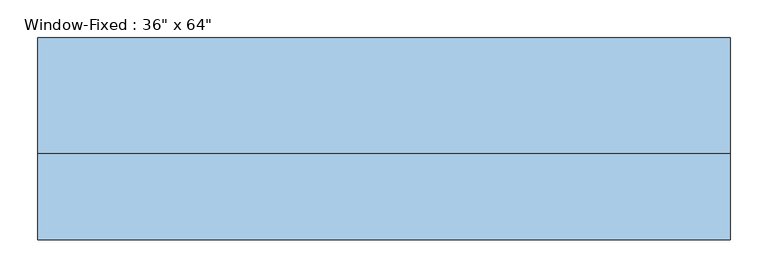
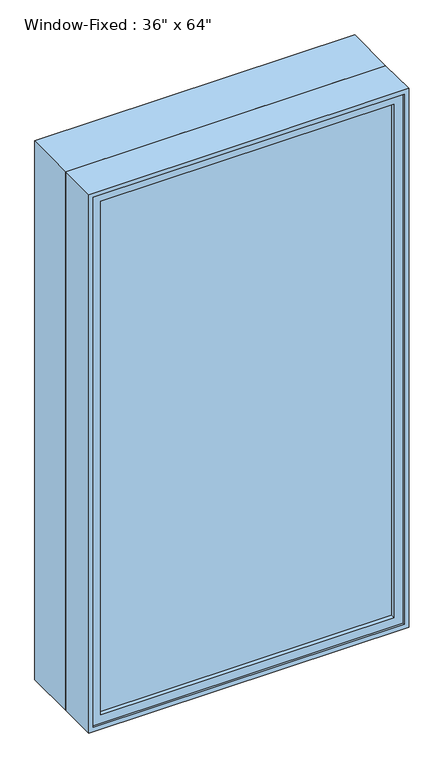
"""IFC4 building model written with IfcOpenShell, lengths in millimetres: window geometry."""

import ifcopenshell
import ifcopenshell.guid

model = None  # the IFC model being written
_history = None  # IfcOwnerHistory: only IFC2X3 demands one
_inside = {}  # id of a spatial element -> (the spatial element, [elements in it])
_under = {}  # id of a project, library or spatial element -> (it, [spatial elements below it])
_declared = {}  # id of a project -> (the project, [libraries it declares])
_typed = {}  # id of a type object -> (the type object, [elements of that type])
_made_of = {}  # id of a material, layer set ... -> (it, [elements and type objects made of it])


def new_model(schema):
    """Start an empty IFC model of exactly this schema.

    Asked for "IFC4X3", IfcOpenShell would pick the latest addendum, in which some entities
    have other attributes; the version numbers below select the first issue.
    IFC2X3 requires an IfcOwnerHistory on every rooted entity: one is made here for all.
    """
    global model, _history
    if schema == "IFC4X3":
        model = ifcopenshell.file(schema_version=(4, 3, 0, 0))
    else:
        model = ifcopenshell.file(schema=schema)
    _inside.clear()
    _under.clear()
    _declared.clear()
    _typed.clear()
    _made_of.clear()
    _history = None
    if model.schema == "IFC2X3":
        org = make("IfcOrganization", Name="unknown")
        user = make(
            "IfcPersonAndOrganization",
            ThePerson=make("IfcPerson", FamilyName="unknown"),
            TheOrganization=org,
        )
        app = make(
            "IfcApplication",
            ApplicationDeveloper=org,
            Version="unknown",
            ApplicationFullName="unknown",
            ApplicationIdentifier="unknown",
        )
        _history = make(
            "IfcOwnerHistory",
            OwningUser=user,
            OwningApplication=app,
            ChangeAction="ADDED",
            CreationDate=0,
        )
    return model


def make(cls, **values):
    """One entity of the class cls with the attributes given. An attribute that is None is left unset."""
    return model.create_entity(
        cls, **{name: value for name, value in values.items() if value is not None}
    )


def rooted(cls, **values):
    """An entity with a GlobalId (a new one), such as an element, a storey or a relation."""
    return make(cls, GlobalId=ifcopenshell.guid.new(), OwnerHistory=_history, **values)


def si_unit(unit_type, name, prefix=None):
    """IfcSIUnit, for example si_unit("LENGTHUNIT", "METRE", prefix="MILLI")."""
    return make("IfcSIUnit", UnitType=unit_type, Prefix=prefix, Name=name)


def assignment(units):
    """IfcUnitAssignment: the units of a project."""
    return None if units is None else make("IfcUnitAssignment", Units=units)


def point(xyz):
    """IfcCartesianPoint."""
    return None if xyz is None else make("IfcCartesianPoint", Coordinates=xyz)


def direction(xyz):
    """IfcDirection."""
    return None if xyz is None else make("IfcDirection", DirectionRatios=xyz)


def frame(location, z_axis=None, x_axis=None):
    """IfcAxis2Placement3D, a coordinate frame: its origin and axes. An axis left out is left unset."""
    return make(
        "IfcAxis2Placement3D",
        Location=point(location),
        Axis=direction(z_axis),
        RefDirection=direction(x_axis),
    )


def origin():
    """The frame at (0, 0, 0) with its axes left unset."""
    return frame((0.0, 0.0, 0.0))


def place(relative_to, where):
    """IfcLocalPlacement: puts the frame where relative to a parent placement (None: the world)."""
    return make(
        "IfcLocalPlacement", PlacementRelTo=relative_to, RelativePlacement=where
    )


def context(
    kind, dimensions, precision=None, world=None, true_north=None, identifier=None
):
    """IfcGeometricRepresentationContext, for example the 3D "Model" context."""
    return make(
        "IfcGeometricRepresentationContext",
        ContextIdentifier=identifier,
        ContextType=kind,
        CoordinateSpaceDimension=dimensions,
        Precision=precision,
        WorldCoordinateSystem=world,
        TrueNorth=true_north,
    )


def project(units=None, contexts=None):
    """IfcProject with its units and contexts."""
    return rooted(
        "IfcProject",
        Name="project",
        RepresentationContexts=contexts,
        UnitsInContext=assignment(units),
    )


def spatial(cls, under=None, at=None, **own):
    """A site, building, storey or space (cls), placed at a placement, below another one or the project."""
    s = rooted(cls, ObjectPlacement=at, **own)
    if under is not None:
        _under.setdefault(under.id(), (under, []))[1].append(s)
    return s


def polyline(points):
    """IfcPolyline through the points."""
    return make("IfcPolyline", Points=[point(p) for p in points])


def outline(outer, holes=None, kind="AREA"):
    """IfcArbitraryClosedProfileDef: a profile drawn as a closed curve; with holes, ...WithVoids."""
    if holes is None:
        return make("IfcArbitraryClosedProfileDef", ProfileType=kind, OuterCurve=outer)
    return make(
        "IfcArbitraryProfileDefWithVoids",
        ProfileType=kind,
        OuterCurve=outer,
        InnerCurves=holes,
    )


def extrude(swept, where, along, depth):
    """IfcExtrudedAreaSolid: the profile swept, set in the frame where, extruded along a direction by depth."""
    return make(
        "IfcExtrudedAreaSolid",
        SweptArea=swept,
        Position=where,
        ExtrudedDirection=direction(along),
        Depth=depth,
    )


def faces_of(points, faces, orient=None, outer=None):
    """IfcFace entities. A face is a list of loops; a loop is a list of indices into points, from 0.

    orient and outer hold one flag for each loop. By default every Orientation is true, the
    first loop of a face is its IfcFaceOuterBound and the others are IfcFaceBound.
    """
    made = []
    for i, loops in enumerate(faces):
        bounds = []
        for j, loop in enumerate(loops):
            is_outer = j == 0 if outer is None else outer[i][j]
            bounds.append(
                make(
                    "IfcFaceOuterBound" if is_outer else "IfcFaceBound",
                    Bound=make("IfcPolyLoop", Polygon=[points[k] for k in loop]),
                    Orientation=True if orient is None else orient[i][j],
                )
            )
        made.append(make("IfcFace", Bounds=bounds))
    return made


def faceted_brep(points, faces, orient=None, outer=None, voids=None):
    """IfcFacetedBrep: a solid bounded by flat faces; with voids (closed shells), ...WithVoids."""
    shared = [point(p) for p in points]
    hull = make("IfcClosedShell", CfsFaces=faces_of(shared, faces, orient, outer))
    if voids is None:
        return make("IfcFacetedBrep", Outer=hull)
    return make(
        "IfcFacetedBrepWithVoids",
        Outer=hull,
        Voids=[
            make(cls, CfsFaces=faces_of(shared, fs, o, b)) for cls, fs, o, b in voids
        ],
    )


def shape(context_of_items, identifier, shape_type, items):
    """IfcShapeRepresentation: the items that make up one representation, for example the "Body"."""
    return make(
        "IfcShapeRepresentation",
        ContextOfItems=context_of_items,
        RepresentationIdentifier=identifier,
        RepresentationType=shape_type,
        Items=items,
    )


def source(mapping_origin, context_of_items, identifier, shape_type, items):
    """IfcRepresentationMap: a shape defined once, which mapped items show again and again."""
    return make(
        "IfcRepresentationMap",
        MappingOrigin=mapping_origin,
        MappedRepresentation=shape(context_of_items, identifier, shape_type, items),
    )


def transform(
    local_origin,
    x_axis=None,
    y_axis=None,
    z_axis=None,
    scale=None,
    scale2=None,
    scale3=None,
    uniform=True,
):
    """IfcCartesianTransformationOperator3D, or its non-uniform kind. x_axis, y_axis, z_axis: its Axis1, 2, 3."""
    if uniform:
        return make(
            "IfcCartesianTransformationOperator3D",
            Axis1=direction(x_axis),
            Axis2=direction(y_axis),
            LocalOrigin=point(local_origin),
            Scale=scale,
            Axis3=direction(z_axis),
        )
    return make(
        "IfcCartesianTransformationOperator3DnonUniform",
        Axis1=direction(x_axis),
        Axis2=direction(y_axis),
        LocalOrigin=point(local_origin),
        Scale=scale,
        Axis3=direction(z_axis),
        Scale2=scale2,
        Scale3=scale3,
    )


def mapped(mapping_source, mapping_target):
    """IfcMappedItem: shows the shape of a source again, moved by a transform."""
    return make(
        "IfcMappedItem", MappingSource=mapping_source, MappingTarget=mapping_target
    )


def made_of(thing, what):
    """Note that an element or type object is made of a material, layer set ...; save() writes the relation."""
    if what is not None:
        _made_of.setdefault(what.id(), (what, []))[1].append(thing)
    return thing


def element(
    cls,
    number,
    at=None,
    inside=None,
    cuts=None,
    type_object=None,
    material=None,
    context=None,
    identifier="Body",
    shape_type=None,
    held_by="IfcProductDefinitionShape",
    body=None,
    shapes=None,
    **own,
):
    """One element of the class cls, such as IfcWall. Its Tag is "e" and its number.

    at: its placement. inside: the storey or other place that contains it. cuts: it is an
    opening in that element (IfcRelVoidsElement). A single representation is given by context,
    identifier, shape_type and body (its items); several are given by shapes. held_by: the class
    of the entity that holds the representations. save() writes the other relations.
    """
    e = rooted(cls, Tag="e%d" % number, ObjectPlacement=at, **own)
    if body is not None:
        shapes = [shape(context, identifier, shape_type, body)]
    if shapes is not None:
        e.Representation = make(held_by, Representations=shapes)
    if inside is not None:
        _inside.setdefault(inside.id(), (inside, []))[1].append(e)
    if cuts is not None:
        rooted(
            "IfcRelVoidsElement", RelatingBuildingElement=cuts, RelatedOpeningElement=e
        )
    if type_object is not None:
        _typed.setdefault(type_object.id(), (type_object, []))[1].append(e)
    return made_of(e, material)


def aggregate(whole, parts):
    """IfcRelAggregates: a whole, such as a stair, and the parts it consists of."""
    return rooted("IfcRelAggregates", RelatingObject=whole, RelatedObjects=parts)


def save(model, path):
    """Write the relations noted so far, then the file.

    IfcRelAggregates (storeys below a building ...), IfcRelContainedInSpatialStructure (elements
    in a storey), IfcRelDefinesByType, IfcRelAssociatesMaterial and IfcRelDeclares: one each for
    every whole, place, type object, material and project.
    """
    for whole, parts in _under.values():
        aggregate(whole, parts)
    for where, things in _inside.values():
        rooted(
            "IfcRelContainedInSpatialStructure",
            RelatedElements=things,
            RelatingStructure=where,
        )
    for kind, things in _typed.values():
        rooted("IfcRelDefinesByType", RelatedObjects=things, RelatingType=kind)
    for what, things in _made_of.values():
        rooted("IfcRelAssociatesMaterial", RelatedObjects=things, RelatingMaterial=what)
    for by, libraries in _declared.values():
        rooted("IfcRelDeclares", RelatingContext=by, RelatedDefinitions=libraries)
    model.write(path)


def window_b05dfed1(model_context):
    return source(origin(), model_context, "Body", "SolidModel", [
        extrude(outline(polyline([(419.1, -79.375), (-419.1, -79.375), (-419.1, -73.025), (419.1, -73.025), (419.1, -79.375)])), frame((0.0, 0.0, 952.5), z_axis=(0.0, 0.0, 1.0), x_axis=(1.0, 0.0, 0.0)), (0.0, 0.0, 1.0), 1549.4),
        extrude(outline(polyline([(-419.1, -60.325), (419.1, -60.325), (419.1, -66.675), (-419.1, -66.675), (-419.1, -60.325)])), frame((0.0, 0.0, 952.5), z_axis=(0.0, 0.0, 1.0), x_axis=(1.0, 0.0, 0.0)), (0.0, 0.0, 1.0), 1549.4),
        extrude(outline(polyline([(927.1, -444.5), (927.1, 444.5), (2527.3, 444.5), (2527.3, -444.5), (927.1, -444.5)]), holes=[polyline([(952.5, 419.1), (952.5, -419.1), (2501.9, -419.1), (2501.9, 419.1), (952.5, 419.1)])]), frame((0.0, -92.075, 0.0), z_axis=(0.0, 1.0, 0.0), x_axis=(0.0, 0.0, 1.0)), (0.0, 0.0, 1.0), 44.45),
        extrude(outline(polyline([(2540.0, -457.2), (914.4, -457.2), (914.4, 457.2), (2540.0, 457.2), (2540.0, -457.2)]), holes=[polyline([(2527.3, 444.5), (927.1, 444.5), (927.1, -444.5), (2527.3, -444.5), (2527.3, 444.5)])]), frame((0.0, 15.875, 0.0), z_axis=(0.0, 1.0, 0.0), x_axis=(0.0, 0.0, 1.0)), (0.0, 0.0, 1.0), 152.4),
        faceted_brep([(457.2, 15.875, 2540.0), (-457.2, 15.875, 2540.0), (-457.2, -98.425, 2540.0), (457.2, -98.425, 2540.0), (-457.2, 15.875, 914.4), (-457.2, -98.425, 914.4), (457.2, 15.875, 914.4), (457.2, -98.425, 914.4), (425.45, 15.875, 2508.25), (-425.45, 15.875, 2508.25), (-425.45, 15.875, 946.15), (425.45, 15.875, 946.15), (-444.5, -98.425, 2527.3), (444.5, -98.425, 2527.3), (444.5, -98.425, 927.1), (-444.5, -98.425, 927.1), (425.45, -47.625, 2508.25), (-425.45, -47.625, 2508.25), (-444.5, -47.625, 2527.3), (444.5, -47.625, 2527.3), (-425.45, -47.625, 946.15), (-444.5, -47.625, 927.1), (425.45, -47.625, 946.15), (444.5, -47.625, 927.1)], [[[0, 1, 2, 3]], [[1, 4, 5, 2]], [[4, 6, 7, 5]], [[1, 0, 6, 4], [8, 9, 10, 11]], [[6, 0, 3, 7]], [[3, 2, 5, 7], [12, 13, 14, 15]], [[16, 17, 9, 8]], [[13, 12, 18, 19]], [[17, 20, 10, 9]], [[12, 15, 21, 18]], [[20, 22, 11, 10]], [[15, 14, 23, 21]], [[22, 16, 8, 11]], [[19, 18, 21, 23], [17, 16, 22, 20]], [[14, 13, 19, 23]]]),
    ])


if __name__ == "__main__":
    model = new_model("IFC4")
    model_context = context("Model", 3, world=origin())
    ifc_project = project(units=[si_unit("LENGTHUNIT", "METRE", prefix="MILLI")], contexts=[model_context])
    site = spatial("IfcSite", under=ifc_project)
    building = spatial("IfcBuilding", under=site)
    placement = place(None, origin())
    window_shape = window_b05dfed1(model_context)
    element("IfcWindow", 1, ObjectType="Window-Fixed : 36\" x 64\"", at=placement, inside=building, context=model_context, shape_type="MappedRepresentation", body=[
        mapped(window_shape, transform((0.0, 0.0, 0.0), x_axis=(1.0, 0.0, 0.0), y_axis=(0.0, 1.0, 0.0), z_axis=(0.0, 0.0, 1.0))),
    ])
    save(model, "model.ifc")

# Revit data of these elements
# Type "Window-Fixed : 36\" x 64\""
#   Type Mark = "23"
#   Fire Rating = "0.5h"
#   Assembly Code = "B2020100"
#   Analytic Construction = "Double glazing - domestic"
#   Window Inset [instance default] = 0' - 0"
#   Wall Thickness [instance default] = 0' - 6"
#   Visual Light Transmittance = 0.81
#   Thermal Resistance (R) = 1.8146 (h·ft²·°F)/BTU
#   Solar Heat Gain Coefficient = 0.76
#   Rough Width = 3' - 0 1/2"
#   Rough Height = 5' - 4 1/2"
#   Interior Wall Closure [instance default] = 0' - 2 1/4"
#   Height = 5' - 4"
#   Heat Transfer Coefficient (U) = 0.5511 BTU/(h·ft²·°F)
#   Frame Extension [instance default] = 0' - 0 1/4"
#   Exterior Wall Closure [instance default] = 0' - 1 1/4"
#   Extension Jamb [instance default] = 0' - 2 1/4"
#   Default Sill Height = 3' - 0"
#   Width = 3' - 0"
#   Muntin Visibility = yes
#   Interior Trim Visibility [instance default] = yes
#   Exterior Trim Visibility [instance default] = yes
#   Extension Jamb Visibility [instance default] = yes
#   Muntin Pattern = Muntin Pattern_2x2 : Muntin Pattern_2x2
#   Interior Trim Material = Wood - Stained
#   Interior Trim = Trim-Window-Interior-Flat : Picture Frame
#   Interior Frame Material = Wood - Stained
#   Glass Panel Material = Glass
#   Exterior Trim Material = Clad - White
#   Exterior Trim = Trim-Window-Exterior-Flat : with Sill
#   Exterior Frame Material = Clad - White
#   Wall Closure = (empty or 0)
# Element 1 (IfcWindow, "Window-Fixed : 36\" x 64\"")
#   Window Inset = 0' - 3 1/2"
#   Wall Thickness = 1' - 1 1/4"
#   Exterior Wall Closure = 0' - 5 1/2"
#   Extension Jamb = 0' - 6"
#   Exterior Trim Visibility = no
#   Materials on its faces: "Wood - Stained", "Glass", "Clad - White"
# Materials
#   "Wood - Stained": class "Wood", colour RGB 224 178 126, transparency 0, Cost = 0
#   "Glass": class "Glass", colour RGB 0 128 192, transparency 0.75, Description = "Soda Lime Glass", Cost = 0
#   "Clad - White": class "Wood", colour RGB 242 242 238, transparency 0, Cost = 0
